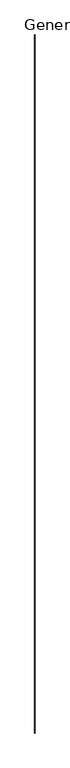
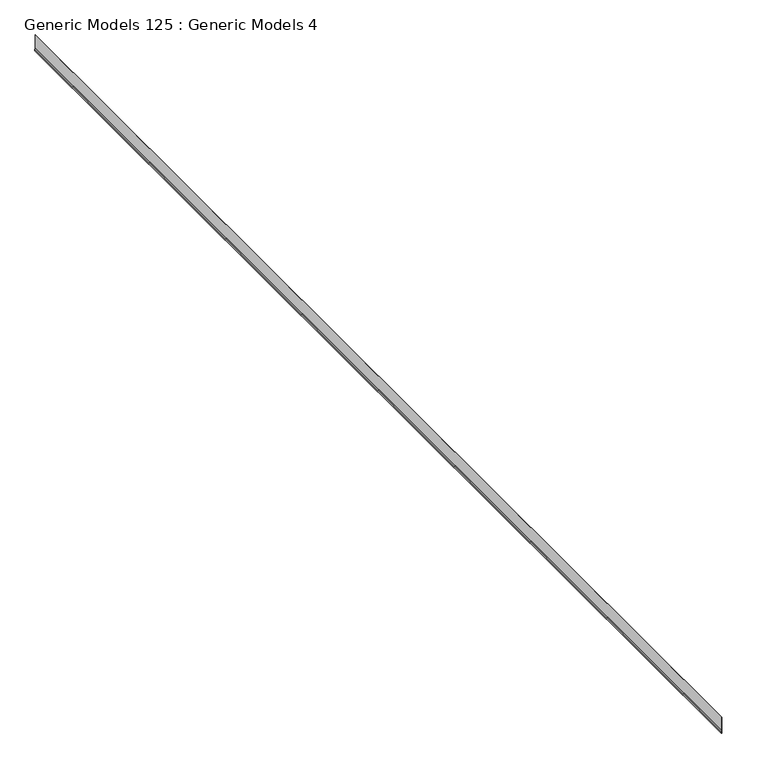
"""IFC4 building model written with IfcOpenShell, lengths in millimetres: proxy geometry, Generic Models 125 : Generic Models 4."""

import ifcopenshell
import ifcopenshell.guid

model = None  # the IFC model being written
_history = None  # IfcOwnerHistory: only IFC2X3 demands one
_inside = {}  # id of a spatial element -> (the spatial element, [elements in it])
_under = {}  # id of a project, library or spatial element -> (it, [spatial elements below it])
_declared = {}  # id of a project -> (the project, [libraries it declares])
_typed = {}  # id of a type object -> (the type object, [elements of that type])
_made_of = {}  # id of a material, layer set ... -> (it, [elements and type objects made of it])


def new_model(schema):
    """Start an empty IFC model of exactly this schema.

    Asked for "IFC4X3", IfcOpenShell would pick the latest addendum, in which some entities
    have other attributes; the version numbers below select the first issue.
    IFC2X3 requires an IfcOwnerHistory on every rooted entity: one is made here for all.
    """
    global model, _history
    if schema == "IFC4X3":
        model = ifcopenshell.file(schema_version=(4, 3, 0, 0))
    else:
        model = ifcopenshell.file(schema=schema)
    _inside.clear()
    _under.clear()
    _declared.clear()
    _typed.clear()
    _made_of.clear()
    _history = None
    if model.schema == "IFC2X3":
        org = make("IfcOrganization", Name="unknown")
        user = make(
            "IfcPersonAndOrganization",
            ThePerson=make("IfcPerson", FamilyName="unknown"),
            TheOrganization=org,
        )
        app = make(
            "IfcApplication",
            ApplicationDeveloper=org,
            Version="unknown",
            ApplicationFullName="unknown",
            ApplicationIdentifier="unknown",
        )
        _history = make(
            "IfcOwnerHistory",
            OwningUser=user,
            OwningApplication=app,
            ChangeAction="ADDED",
            CreationDate=0,
        )
    return model


def make(cls, **values):
    """One entity of the class cls with the attributes given. An attribute that is None is left unset."""
    return model.create_entity(
        cls, **{name: value for name, value in values.items() if value is not None}
    )


def rooted(cls, **values):
    """An entity with a GlobalId (a new one), such as an element, a storey or a relation."""
    return make(cls, GlobalId=ifcopenshell.guid.new(), OwnerHistory=_history, **values)


def si_unit(unit_type, name, prefix=None):
    """IfcSIUnit, for example si_unit("LENGTHUNIT", "METRE", prefix="MILLI")."""
    return make("IfcSIUnit", UnitType=unit_type, Prefix=prefix, Name=name)


def assignment(units):
    """IfcUnitAssignment: the units of a project."""
    return None if units is None else make("IfcUnitAssignment", Units=units)


def point(xyz):
    """IfcCartesianPoint."""
    return None if xyz is None else make("IfcCartesianPoint", Coordinates=xyz)


def direction(xyz):
    """IfcDirection."""
    return None if xyz is None else make("IfcDirection", DirectionRatios=xyz)


def frame(location, z_axis=None, x_axis=None):
    """IfcAxis2Placement3D, a coordinate frame: its origin and axes. An axis left out is left unset."""
    return make(
        "IfcAxis2Placement3D",
        Location=point(location),
        Axis=direction(z_axis),
        RefDirection=direction(x_axis),
    )


def origin():
    """The frame at (0, 0, 0) with its axes left unset."""
    return frame((0.0, 0.0, 0.0))


def place(relative_to, where):
    """IfcLocalPlacement: puts the frame where relative to a parent placement (None: the world)."""
    return make(
        "IfcLocalPlacement", PlacementRelTo=relative_to, RelativePlacement=where
    )


def context(
    kind, dimensions, precision=None, world=None, true_north=None, identifier=None
):
    """IfcGeometricRepresentationContext, for example the 3D "Model" context."""
    return make(
        "IfcGeometricRepresentationContext",
        ContextIdentifier=identifier,
        ContextType=kind,
        CoordinateSpaceDimension=dimensions,
        Precision=precision,
        WorldCoordinateSystem=world,
        TrueNorth=true_north,
    )


def project(units=None, contexts=None):
    """IfcProject with its units and contexts."""
    return rooted(
        "IfcProject",
        Name="project",
        RepresentationContexts=contexts,
        UnitsInContext=assignment(units),
    )


def spatial(cls, under=None, at=None, **own):
    """A site, building, storey or space (cls), placed at a placement, below another one or the project."""
    s = rooted(cls, ObjectPlacement=at, **own)
    if under is not None:
        _under.setdefault(under.id(), (under, []))[1].append(s)
    return s


def polyline(points):
    """IfcPolyline through the points."""
    return make("IfcPolyline", Points=[point(p) for p in points])


def outline(outer, holes=None, kind="AREA"):
    """IfcArbitraryClosedProfileDef: a profile drawn as a closed curve; with holes, ...WithVoids."""
    if holes is None:
        return make("IfcArbitraryClosedProfileDef", ProfileType=kind, OuterCurve=outer)
    return make(
        "IfcArbitraryProfileDefWithVoids",
        ProfileType=kind,
        OuterCurve=outer,
        InnerCurves=holes,
    )


def extrude(swept, where, along, depth):
    """IfcExtrudedAreaSolid: the profile swept, set in the frame where, extruded along a direction by depth."""
    return make(
        "IfcExtrudedAreaSolid",
        SweptArea=swept,
        Position=where,
        ExtrudedDirection=direction(along),
        Depth=depth,
    )


def shape(context_of_items, identifier, shape_type, items):
    """IfcShapeRepresentation: the items that make up one representation, for example the "Body"."""
    return make(
        "IfcShapeRepresentation",
        ContextOfItems=context_of_items,
        RepresentationIdentifier=identifier,
        RepresentationType=shape_type,
        Items=items,
    )


def source(mapping_origin, context_of_items, identifier, shape_type, items):
    """IfcRepresentationMap: a shape defined once, which mapped items show again and again."""
    return make(
        "IfcRepresentationMap",
        MappingOrigin=mapping_origin,
        MappedRepresentation=shape(context_of_items, identifier, shape_type, items),
    )


def transform(
    local_origin,
    x_axis=None,
    y_axis=None,
    z_axis=None,
    scale=None,
    scale2=None,
    scale3=None,
    uniform=True,
):
    """IfcCartesianTransformationOperator3D, or its non-uniform kind. x_axis, y_axis, z_axis: its Axis1, 2, 3."""
    if uniform:
        return make(
            "IfcCartesianTransformationOperator3D",
            Axis1=direction(x_axis),
            Axis2=direction(y_axis),
            LocalOrigin=point(local_origin),
            Scale=scale,
            Axis3=direction(z_axis),
        )
    return make(
        "IfcCartesianTransformationOperator3DnonUniform",
        Axis1=direction(x_axis),
        Axis2=direction(y_axis),
        LocalOrigin=point(local_origin),
        Scale=scale,
        Axis3=direction(z_axis),
        Scale2=scale2,
        Scale3=scale3,
    )


def mapped(mapping_source, mapping_target):
    """IfcMappedItem: shows the shape of a source again, moved by a transform."""
    return make(
        "IfcMappedItem", MappingSource=mapping_source, MappingTarget=mapping_target
    )


def made_of(thing, what):
    """Note that an element or type object is made of a material, layer set ...; save() writes the relation."""
    if what is not None:
        _made_of.setdefault(what.id(), (what, []))[1].append(thing)
    return thing


def element(
    cls,
    number,
    at=None,
    inside=None,
    cuts=None,
    type_object=None,
    material=None,
    context=None,
    identifier="Body",
    shape_type=None,
    held_by="IfcProductDefinitionShape",
    body=None,
    shapes=None,
    **own,
):
    """One element of the class cls, such as IfcWall. Its Tag is "e" and its number.

    at: its placement. inside: the storey or other place that contains it. cuts: it is an
    opening in that element (IfcRelVoidsElement). A single representation is given by context,
    identifier, shape_type and body (its items); several are given by shapes. held_by: the class
    of the entity that holds the representations. save() writes the other relations.
    """
    e = rooted(cls, Tag="e%d" % number, ObjectPlacement=at, **own)
    if body is not None:
        shapes = [shape(context, identifier, shape_type, body)]
    if shapes is not None:
        e.Representation = make(held_by, Representations=shapes)
    if inside is not None:
        _inside.setdefault(inside.id(), (inside, []))[1].append(e)
    if cuts is not None:
        rooted(
            "IfcRelVoidsElement", RelatingBuildingElement=cuts, RelatedOpeningElement=e
        )
    if type_object is not None:
        _typed.setdefault(type_object.id(), (type_object, []))[1].append(e)
    return made_of(e, material)


def aggregate(whole, parts):
    """IfcRelAggregates: a whole, such as a stair, and the parts it consists of."""
    return rooted("IfcRelAggregates", RelatingObject=whole, RelatedObjects=parts)


def save(model, path):
    """Write the relations noted so far, then the file.

    IfcRelAggregates (storeys below a building ...), IfcRelContainedInSpatialStructure (elements
    in a storey), IfcRelDefinesByType, IfcRelAssociatesMaterial and IfcRelDeclares: one each for
    every whole, place, type object, material and project.
    """
    for whole, parts in _under.values():
        aggregate(whole, parts)
    for where, things in _inside.values():
        rooted(
            "IfcRelContainedInSpatialStructure",
            RelatedElements=things,
            RelatingStructure=where,
        )
    for kind, things in _typed.values():
        rooted("IfcRelDefinesByType", RelatedObjects=things, RelatingType=kind)
    for what, things in _made_of.values():
        rooted("IfcRelAssociatesMaterial", RelatedObjects=things, RelatingMaterial=what)
    for by, libraries in _declared.values():
        rooted("IfcRelDeclares", RelatingContext=by, RelatedDefinitions=libraries)
    model.write(path)


def generic_models_125_generic_models_4_b2147425(model_context):
    return source(origin(), model_context, "Body", "SweptSolid", [
        extrude(outline(polyline([(126222.1824536, -6624.0173796), (126364.746, -6624.0173796), (126364.746, -6624.8111296), (126222.3224132, -6624.8111296), (126211.2286669, -6628.848923), (126196.1749044, -6628.848923), (126196.1749044, -6628.055173), (126211.0887074, -6628.055173), (126222.1824536, -6624.0173796)])), frame((0.0, -464.1230338, 0.0), z_axis=(0.0, 1.0, 0.0), x_axis=(0.0, 0.0, 1.0)), (0.0, 0.0, 1.0), 12242.8),
    ])


if __name__ == "__main__":
    model = new_model("IFC4")
    model_context = context("Model", 3, world=origin())
    ifc_project = project(units=[si_unit("LENGTHUNIT", "METRE", prefix="MILLI")], contexts=[model_context])
    site = spatial("IfcSite", under=ifc_project)
    building = spatial("IfcBuilding", under=site)
    placement = place(None, origin())
    generic_models_125_generic_models_4_shape = generic_models_125_generic_models_4_b2147425(model_context)
    element("IfcBuildingElementProxy", 1, Name="Generic Models 125 : Generic Models 4", ObjectType="Generic Models 125 : Generic Models 4", at=placement, inside=building, context=model_context, shape_type="MappedRepresentation", body=[
        mapped(generic_models_125_generic_models_4_shape, transform((0.0, 0.0, 0.0), x_axis=(1.0, 0.0, 0.0), y_axis=(0.0, 1.0, 0.0), z_axis=(0.0, 0.0, 1.0))),
    ])
    save(model, "model.ifc")

# Revit data of these elements
# Element 1 (IfcBuildingElementProxy, "Generic Models 125 : Generic Models 4")
#   Materials on its faces: "_(2) LAYERS NO. 30 ASTM D226 ASPHALT SATURATED ORGANIC FELT"
# Materials
#   "_(2) LAYERS NO. 30 ASTM D226 ASPHALT SATURATED ORGANIC FELT": class "Generic", colour RGB 67 154 161, transparency 0, Cost = 0
